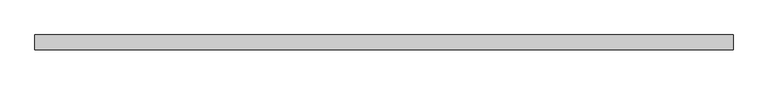
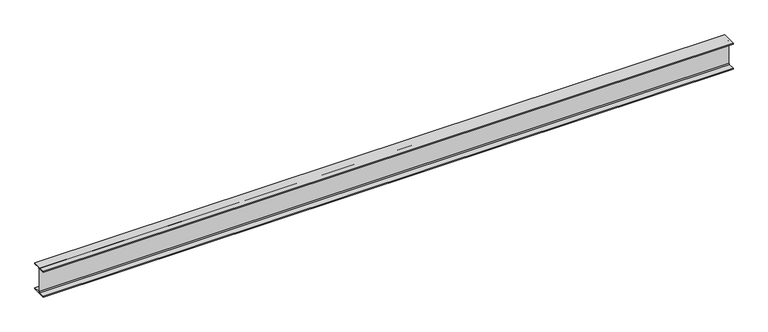
"""IFC4 building model written with IfcOpenShell, lengths in millimetres: beam geometry, Old_Steel Beam_H-KSD3502 : H_SB_ASB_H-340×250x9x14."""

from ifc_helpers import new_model, si_unit, point, frame, frame_2d, origin, place, context, project, spatial, polyline, circle_curve, trimmed, segment, composite_curve, outline, extrude, source, transform, mapped, element, save


def beam_3c5e3aa6(model_context):
    return source(origin(), model_context, "Body", "SweptSolid", [
        extrude(outline(composite_curve([segment(polyline([(82.5, -141.5), (82.5, -151.7), (-82.5, -151.7), (-82.5, -141.5), (-11.9, -141.5)]), True, "CONTINUOUS"), segment(trimmed(circle_curve(frame_2d((-11.9, -132.6)), 8.9), [point((-11.9, -141.5))], [point((-3.0, -132.6))], True, "CARTESIAN"), True, "CONTINUOUS"), segment(polyline([(-3.0, -132.6), (-3.0, 132.6)]), True, "CONTINUOUS"), segment(trimmed(circle_curve(frame_2d((-11.9, 132.6)), 8.9), [point((-3.0, 132.6))], [point((-11.9, 141.5))], True, "CARTESIAN"), True, "CONTINUOUS"), segment(polyline([(-11.9, 141.5), (-82.5, 141.5), (-82.5, 151.7), (82.5, 151.7), (82.5, 141.5), (11.9, 141.5)]), True, "CONTINUOUS"), segment(trimmed(circle_curve(frame_2d((11.9, 132.6)), 8.9), [point((11.9, 141.5))], [point((3.0, 132.6))], True, "CARTESIAN"), True, "CONTINUOUS"), segment(polyline([(3.0, 132.6), (3.0, -132.6)]), True, "CONTINUOUS"), segment(trimmed(circle_curve(frame_2d((11.9, -132.6)), 8.9), [point((3.0, -132.6))], [point((11.9, -141.5))], True, "CARTESIAN"), True, "CONTINUOUS"), segment(polyline([(11.9, -141.5), (82.5, -141.5)]), True, "CONTINUOUS")], self_intersect=False)), frame((-3837.3, 0.0, 0.0), z_axis=(1.0, 0.0, 0.0), x_axis=(0.0, 1.0, 0.0)), (0.0, 0.0, 1.0), 7674.6),
    ])


if __name__ == "__main__":
    model = new_model("IFC4")
    model_context = context("Model", 3, world=origin())
    ifc_project = project(units=[si_unit("LENGTHUNIT", "METRE", prefix="MILLI")], contexts=[model_context])
    site = spatial("IfcSite", under=ifc_project)
    building = spatial("IfcBuilding", under=site)
    placement = place(None, origin())
    beam_shape = beam_3c5e3aa6(model_context)
    element("IfcBeam", 1, ObjectType="Old_Steel Beam_H-KSD3502 : H_SB_ASB_H-340×250x9x14", at=placement, inside=building, context=model_context, shape_type="MappedRepresentation", body=[
        mapped(beam_shape, transform((0.0, 0.0, 0.0), x_axis=(1.0, 0.0, 0.0), y_axis=(0.0, 1.0, 0.0), z_axis=(0.0, 0.0, 1.0))),
    ])
    save(model, "model.ifc")

# Revit data of these elements
# Type "Old_Steel Beam_H-KSD3502 : H_SB_ASB_H-340×250x9x14"
#   Width = 25.0 cm
#   Web Thickness = 0.9 cm
#   Web Fillet = 2.0 cm
#   Warping Constant = 968661.0 cm⁶
#   Torsional Moment of Inertia = 53.6551 cm⁴
#   Torsional Modulus = 1.0 cm³
#   Section Area = 101.5 cm²
#   Plastic Modulus weak axis = 447.0 cm³
#   Plastic Modulus strong axis = 1410.0 cm³
#   Perimeter = 1.63 m²/m
#   Nominal Weight = 79.70 kgf/m
#   Moment of Inertia weak axis = 3650.00 cm⁴
#   Moment of Inertia strong axis = 21700.00 cm⁴
#   Height = 34.0 cm
#   Flange Thickness = 1.4 cm
#   Elastic Modulus weak axis = 292.0 cm³
#   Elastic Modulus strong axis = 1280.0 cm³
#   Centroid Vertical = 17.0 cm
#   Centroid Horizontal = 12.5 cm
#   Length [instance default] = 1.5240 m
#   Structural Material [instance default] = Steel, 45-345
#   Assembly Code = ""
# Element 1 (IfcBeam, "Old_Steel Beam_H-KSD3502 : H_SB_ASB_H-340×250x9x14")
#   Structural Material = none
# Materials
#   "Steel, 45-345": class "Metal", colour RGB 189 187 185, transparency 0, Description = "Steel 345 MPa", Cost = 0
